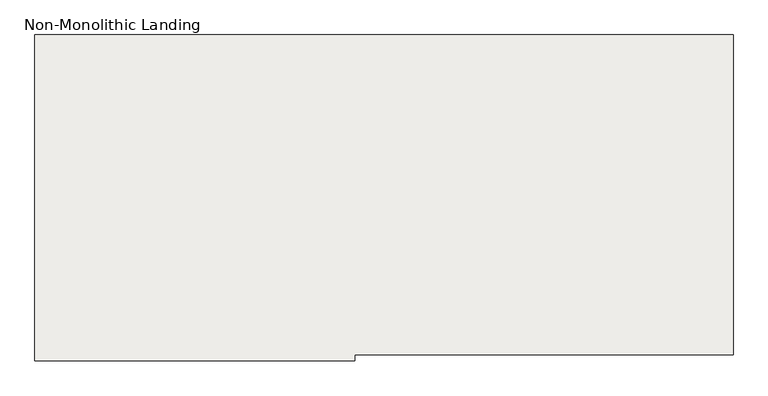
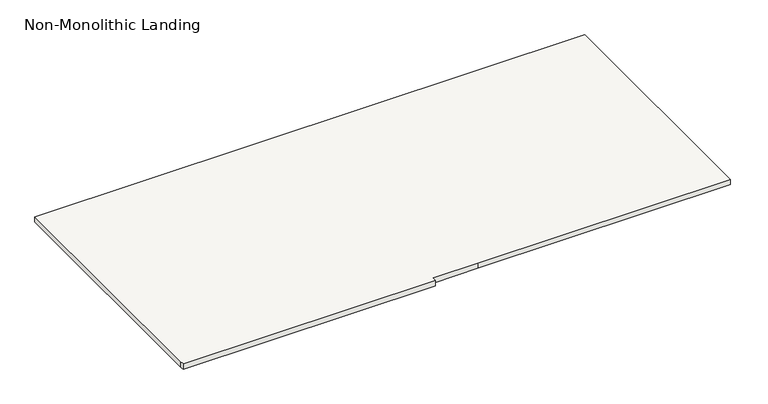
"""IFC4 building model written with IfcOpenShell, lengths in millimetres: slab geometry, Non-Monolithic Landing."""

from ifc_helpers import new_model, si_unit, frame, origin, place, context, project, spatial, polyline, outline, extrude, source, transform, mapped, element, save


def non_monolithic_landing_55c0a7d8(model_context):
    return source(origin(), model_context, "Body", "SweptSolid", [
        extrude(outline(polyline([(-22683.4414763, -9454.4070712), (-22877.1164763, -9454.4070712), (-22877.1164763, -9473.4570712), (-23943.9164763, -9473.4570712), (-23943.9164763, -9454.4070712), (-23943.9164763, -8387.6070712), (-21616.6414763, -8387.6070712), (-21616.6414763, -9454.4070712), (-22683.4414763, -9454.4070712)])), frame((0.0, 0.0, 1347.6882813), z_axis=(0.0, 0.0, 1.0), x_axis=(1.0, 0.0, 0.0)), (0.0, 0.0, 1.0), 23.9117188),
    ])


if __name__ == "__main__":
    model = new_model("IFC4")
    model_context = context("Model", 3, world=origin())
    ifc_project = project(units=[si_unit("LENGTHUNIT", "METRE", prefix="MILLI")], contexts=[model_context])
    site = spatial("IfcSite", under=ifc_project)
    building = spatial("IfcBuilding", under=site)
    placement = place(None, origin())
    non_monolithic_landing_shape = non_monolithic_landing_55c0a7d8(model_context)
    element("IfcSlab", 1, ObjectType="Non-Monolithic Landing", at=placement, inside=building, context=model_context, shape_type="MappedRepresentation", body=[
        mapped(non_monolithic_landing_shape, transform((0.0, 0.0, 0.0), x_axis=(1.0, 0.0, 0.0), y_axis=(0.0, 1.0, 0.0), z_axis=(0.0, 0.0, 1.0))),
    ])
    save(model, "model.ifc")

# Revit data of these elements
# Element 1 (IfcSlab, "Non-Monolithic Landing")
#   Materials on its faces: "Composite Deck - Trex - Select - 1x6 Square Edge Board - Saddle - 20'"
# Materials
#   "Composite Deck - Trex - Select - 1x6 Square Edge Board - Saddle - 20'": class "Wood", colour RGB 120 75 45, transparency 0, Keynote = "06 11 00", Model = "Trex Select® Composite Deck 1\" Square Edge Board", Manufacturer = "Trex", URL = "http://www.trex.com/", Description = "1x6 Trex Select® Composite Deck Square Edge Board", Cost = 0
